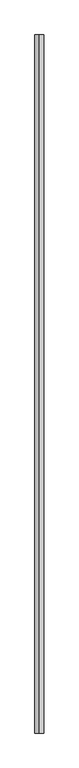
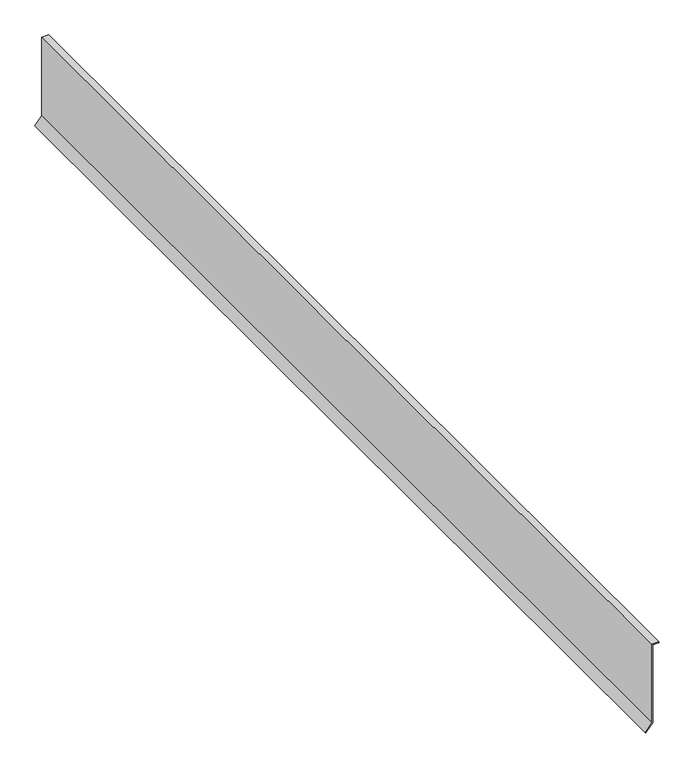
"""IFC4 building model written with IfcOpenShell, lengths in millimetres: proxy geometry, GRAVEL STOP007 14648 : GRAVEL STOP007 14648."""

import ifcopenshell
import ifcopenshell.guid

model = None  # the IFC model being written
_history = None  # IfcOwnerHistory: only IFC2X3 demands one
_inside = {}  # id of a spatial element -> (the spatial element, [elements in it])
_under = {}  # id of a project, library or spatial element -> (it, [spatial elements below it])
_declared = {}  # id of a project -> (the project, [libraries it declares])
_typed = {}  # id of a type object -> (the type object, [elements of that type])
_made_of = {}  # id of a material, layer set ... -> (it, [elements and type objects made of it])


def new_model(schema):
    """Start an empty IFC model of exactly this schema.

    Asked for "IFC4X3", IfcOpenShell would pick the latest addendum, in which some entities
    have other attributes; the version numbers below select the first issue.
    IFC2X3 requires an IfcOwnerHistory on every rooted entity: one is made here for all.
    """
    global model, _history
    if schema == "IFC4X3":
        model = ifcopenshell.file(schema_version=(4, 3, 0, 0))
    else:
        model = ifcopenshell.file(schema=schema)
    _inside.clear()
    _under.clear()
    _declared.clear()
    _typed.clear()
    _made_of.clear()
    _history = None
    if model.schema == "IFC2X3":
        org = make("IfcOrganization", Name="unknown")
        user = make(
            "IfcPersonAndOrganization",
            ThePerson=make("IfcPerson", FamilyName="unknown"),
            TheOrganization=org,
        )
        app = make(
            "IfcApplication",
            ApplicationDeveloper=org,
            Version="unknown",
            ApplicationFullName="unknown",
            ApplicationIdentifier="unknown",
        )
        _history = make(
            "IfcOwnerHistory",
            OwningUser=user,
            OwningApplication=app,
            ChangeAction="ADDED",
            CreationDate=0,
        )
    return model


def make(cls, **values):
    """One entity of the class cls with the attributes given. An attribute that is None is left unset."""
    return model.create_entity(
        cls, **{name: value for name, value in values.items() if value is not None}
    )


def rooted(cls, **values):
    """An entity with a GlobalId (a new one), such as an element, a storey or a relation."""
    return make(cls, GlobalId=ifcopenshell.guid.new(), OwnerHistory=_history, **values)


def si_unit(unit_type, name, prefix=None):
    """IfcSIUnit, for example si_unit("LENGTHUNIT", "METRE", prefix="MILLI")."""
    return make("IfcSIUnit", UnitType=unit_type, Prefix=prefix, Name=name)


def assignment(units):
    """IfcUnitAssignment: the units of a project."""
    return None if units is None else make("IfcUnitAssignment", Units=units)


def point(xyz):
    """IfcCartesianPoint."""
    return None if xyz is None else make("IfcCartesianPoint", Coordinates=xyz)


def direction(xyz):
    """IfcDirection."""
    return None if xyz is None else make("IfcDirection", DirectionRatios=xyz)


def frame(location, z_axis=None, x_axis=None):
    """IfcAxis2Placement3D, a coordinate frame: its origin and axes. An axis left out is left unset."""
    return make(
        "IfcAxis2Placement3D",
        Location=point(location),
        Axis=direction(z_axis),
        RefDirection=direction(x_axis),
    )


def origin():
    """The frame at (0, 0, 0) with its axes left unset."""
    return frame((0.0, 0.0, 0.0))


def place(relative_to, where):
    """IfcLocalPlacement: puts the frame where relative to a parent placement (None: the world)."""
    return make(
        "IfcLocalPlacement", PlacementRelTo=relative_to, RelativePlacement=where
    )


def context(
    kind, dimensions, precision=None, world=None, true_north=None, identifier=None
):
    """IfcGeometricRepresentationContext, for example the 3D "Model" context."""
    return make(
        "IfcGeometricRepresentationContext",
        ContextIdentifier=identifier,
        ContextType=kind,
        CoordinateSpaceDimension=dimensions,
        Precision=precision,
        WorldCoordinateSystem=world,
        TrueNorth=true_north,
    )


def project(units=None, contexts=None):
    """IfcProject with its units and contexts."""
    return rooted(
        "IfcProject",
        Name="project",
        RepresentationContexts=contexts,
        UnitsInContext=assignment(units),
    )


def spatial(cls, under=None, at=None, **own):
    """A site, building, storey or space (cls), placed at a placement, below another one or the project."""
    s = rooted(cls, ObjectPlacement=at, **own)
    if under is not None:
        _under.setdefault(under.id(), (under, []))[1].append(s)
    return s


def polyline(points):
    """IfcPolyline through the points."""
    return make("IfcPolyline", Points=[point(p) for p in points])


def outline(outer, holes=None, kind="AREA"):
    """IfcArbitraryClosedProfileDef: a profile drawn as a closed curve; with holes, ...WithVoids."""
    if holes is None:
        return make("IfcArbitraryClosedProfileDef", ProfileType=kind, OuterCurve=outer)
    return make(
        "IfcArbitraryProfileDefWithVoids",
        ProfileType=kind,
        OuterCurve=outer,
        InnerCurves=holes,
    )


def extrude(swept, where, along, depth):
    """IfcExtrudedAreaSolid: the profile swept, set in the frame where, extruded along a direction by depth."""
    return make(
        "IfcExtrudedAreaSolid",
        SweptArea=swept,
        Position=where,
        ExtrudedDirection=direction(along),
        Depth=depth,
    )


def shape(context_of_items, identifier, shape_type, items):
    """IfcShapeRepresentation: the items that make up one representation, for example the "Body"."""
    return make(
        "IfcShapeRepresentation",
        ContextOfItems=context_of_items,
        RepresentationIdentifier=identifier,
        RepresentationType=shape_type,
        Items=items,
    )


def source(mapping_origin, context_of_items, identifier, shape_type, items):
    """IfcRepresentationMap: a shape defined once, which mapped items show again and again."""
    return make(
        "IfcRepresentationMap",
        MappingOrigin=mapping_origin,
        MappedRepresentation=shape(context_of_items, identifier, shape_type, items),
    )


def transform(
    local_origin,
    x_axis=None,
    y_axis=None,
    z_axis=None,
    scale=None,
    scale2=None,
    scale3=None,
    uniform=True,
):
    """IfcCartesianTransformationOperator3D, or its non-uniform kind. x_axis, y_axis, z_axis: its Axis1, 2, 3."""
    if uniform:
        return make(
            "IfcCartesianTransformationOperator3D",
            Axis1=direction(x_axis),
            Axis2=direction(y_axis),
            LocalOrigin=point(local_origin),
            Scale=scale,
            Axis3=direction(z_axis),
        )
    return make(
        "IfcCartesianTransformationOperator3DnonUniform",
        Axis1=direction(x_axis),
        Axis2=direction(y_axis),
        LocalOrigin=point(local_origin),
        Scale=scale,
        Axis3=direction(z_axis),
        Scale2=scale2,
        Scale3=scale3,
    )


def mapped(mapping_source, mapping_target):
    """IfcMappedItem: shows the shape of a source again, moved by a transform."""
    return make(
        "IfcMappedItem", MappingSource=mapping_source, MappingTarget=mapping_target
    )


def made_of(thing, what):
    """Note that an element or type object is made of a material, layer set ...; save() writes the relation."""
    if what is not None:
        _made_of.setdefault(what.id(), (what, []))[1].append(thing)
    return thing


def element(
    cls,
    number,
    at=None,
    inside=None,
    cuts=None,
    type_object=None,
    material=None,
    context=None,
    identifier="Body",
    shape_type=None,
    held_by="IfcProductDefinitionShape",
    body=None,
    shapes=None,
    **own,
):
    """One element of the class cls, such as IfcWall. Its Tag is "e" and its number.

    at: its placement. inside: the storey or other place that contains it. cuts: it is an
    opening in that element (IfcRelVoidsElement). A single representation is given by context,
    identifier, shape_type and body (its items); several are given by shapes. held_by: the class
    of the entity that holds the representations. save() writes the other relations.
    """
    e = rooted(cls, Tag="e%d" % number, ObjectPlacement=at, **own)
    if body is not None:
        shapes = [shape(context, identifier, shape_type, body)]
    if shapes is not None:
        e.Representation = make(held_by, Representations=shapes)
    if inside is not None:
        _inside.setdefault(inside.id(), (inside, []))[1].append(e)
    if cuts is not None:
        rooted(
            "IfcRelVoidsElement", RelatingBuildingElement=cuts, RelatedOpeningElement=e
        )
    if type_object is not None:
        _typed.setdefault(type_object.id(), (type_object, []))[1].append(e)
    return made_of(e, material)


def aggregate(whole, parts):
    """IfcRelAggregates: a whole, such as a stair, and the parts it consists of."""
    return rooted("IfcRelAggregates", RelatingObject=whole, RelatedObjects=parts)


def save(model, path):
    """Write the relations noted so far, then the file.

    IfcRelAggregates (storeys below a building ...), IfcRelContainedInSpatialStructure (elements
    in a storey), IfcRelDefinesByType, IfcRelAssociatesMaterial and IfcRelDeclares: one each for
    every whole, place, type object, material and project.
    """
    for whole, parts in _under.values():
        aggregate(whole, parts)
    for where, things in _inside.values():
        rooted(
            "IfcRelContainedInSpatialStructure",
            RelatedElements=things,
            RelatingStructure=where,
        )
    for kind, things in _typed.values():
        rooted("IfcRelDefinesByType", RelatedObjects=things, RelatingType=kind)
    for what, things in _made_of.values():
        rooted("IfcRelAssociatesMaterial", RelatedObjects=things, RelatingMaterial=what)
    for by, libraries in _declared.values():
        rooted("IfcRelDeclares", RelatingContext=by, RelatedDefinitions=libraries)
    model.write(path)


def generic_models_a1fe0a36(model_context):
    return source(origin(), model_context, "Body", "SweptSolid", [
        extrude(outline(polyline([(40082.2407116, -2815.6343429), (40081.3605882, -2814.5313394), (40097.4918556, -2801.659661), (40253.3245993, -2801.659661), (40253.3245993, -2789.8917422), (40254.7357103, -2789.8917422), (40254.7357103, -2803.070772), (40097.9858473, -2803.070772), (40082.2407116, -2815.6343429)])), frame((0.0, 999.75, 0.0), z_axis=(0.0, 1.0, 0.0), x_axis=(0.0, 0.0, 1.0)), (0.0, 0.0, 1.0), 2000.25),
    ])


if __name__ == "__main__":
    model = new_model("IFC4")
    model_context = context("Model", 3, world=origin())
    ifc_project = project(units=[si_unit("LENGTHUNIT", "METRE", prefix="MILLI")], contexts=[model_context])
    site = spatial("IfcSite", under=ifc_project)
    building = spatial("IfcBuilding", under=site)
    placement = place(None, origin())
    generic_models_shape = generic_models_a1fe0a36(model_context)
    element("IfcBuildingElementProxy", 1, Name="GRAVEL STOP007 14648 : GRAVEL STOP007 14648", ObjectType="GRAVEL STOP007 14648 : GRAVEL STOP007 14648", at=placement, inside=building, context=model_context, shape_type="MappedRepresentation", body=[
        mapped(generic_models_shape, transform((0.0, 0.0, 0.0), x_axis=(1.0, 0.0, 0.0), y_axis=(0.0, 1.0, 0.0), z_axis=(0.0, 0.0, 1.0))),
    ])
    save(model, "model.ifc")

# Revit data of these elements
# Type "GRAVEL STOP007 14648 : GRAVEL STOP007 14648"
#   NameOverride = "GRAVEL STOP007"
# Element 1 (IfcBuildingElementProxy, "GRAVEL STOP007 14648 : GRAVEL STOP007 14648")
#   Materials on its faces: "GRAVEL STOP REQUIRED WITH GRAVEL SURFACE SYSTEMS"
# Materials
#   "GRAVEL STOP REQUIRED WITH GRAVEL SURFACE SYSTEMS": class "Unassigned", colour RGB 170 170 127, transparency 0
